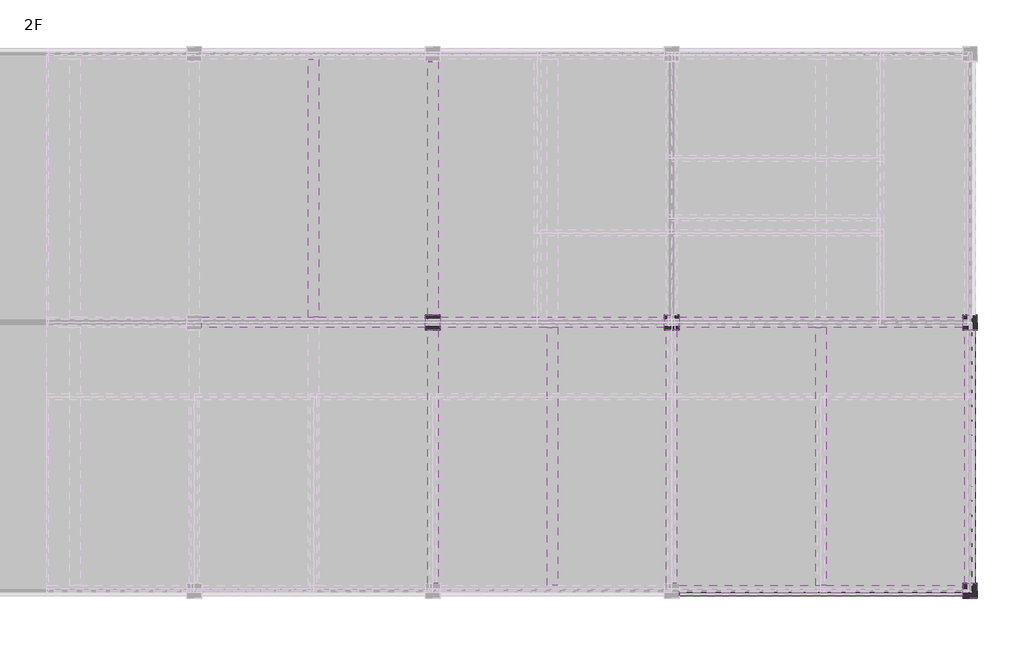
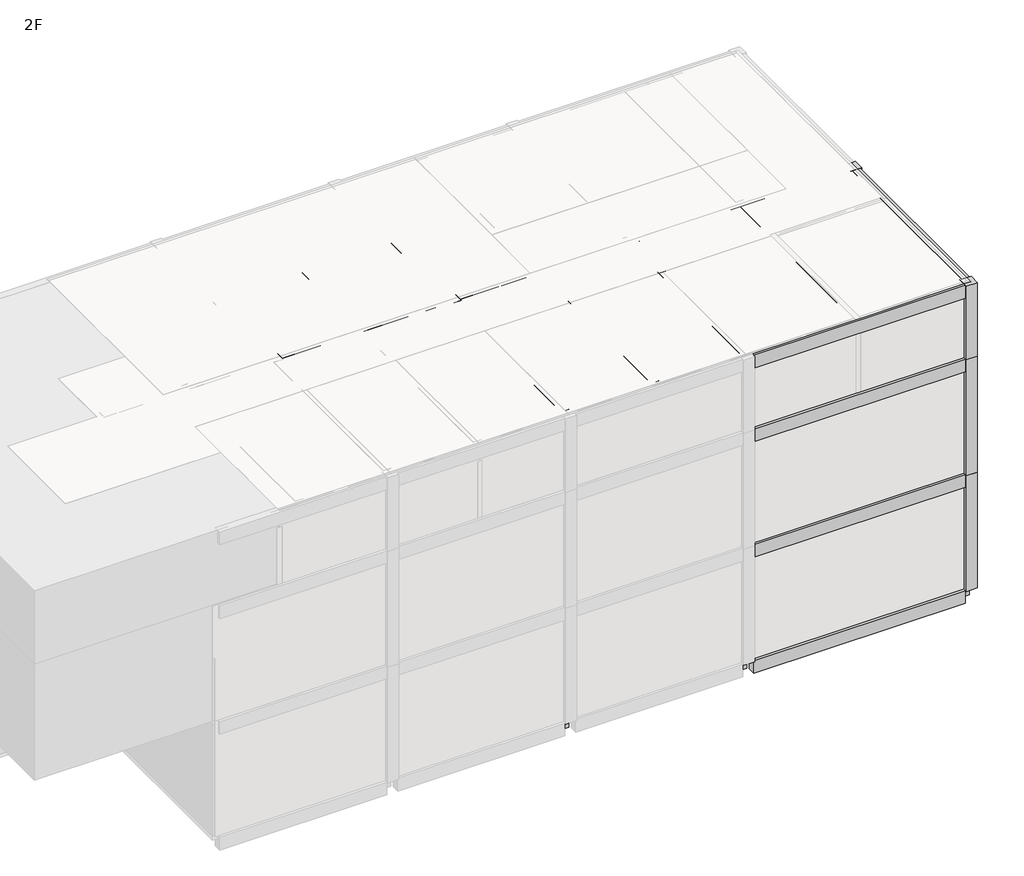
# One storey, part 6 of 7: 44 beams, 12 columns.
"""IFC4 building model written with IfcOpenShell, lengths in millimetres."""

from ifc_helpers import new_model, si_unit, frame, origin, place, context, project, spatial, polyline, outline, extrude, faceted_brep, element, save

model = new_model("IFC4")

# Units and contexts
model_context = context("Model", 3, world=origin())
ifc_project = project(units=[si_unit("LENGTHUNIT", "METRE", prefix="MILLI")], contexts=[model_context])

# Site, building, storey
site = spatial("IfcSite", under=ifc_project)
building = spatial("IfcBuilding", under=site)
storey = spatial("IfcBuildingStorey", under=building, Name="2F", Elevation=3500.0)

# Beams
placement = place(None, origin())
element("IfcBeam", 1, ObjectType="Concrete-Rectangular-Beam : BM111_400x500_RG1", at=placement, inside=storey, context=model_context, shape_type="SweptSolid", body=[
    extrude(outline(polyline([(65634.6521483, 173098.8614395), (65284.6521483, 173098.8614395), (65284.6521483, 181748.8614395), (65634.6521483, 181748.8614395), (65634.6521483, 173098.8614395)])), frame((0.0, 0.0, 2900.0), z_axis=(0.0, 0.0, 1.0), x_axis=(1.0, 0.0, 0.0)), (0.0, 0.0, 1.0), 600.0),
])
element("IfcBeam", 2, ObjectType="Concrete-Rectangular-Beam : BM111_400x500_RG1", at=placement, inside=storey, context=model_context, shape_type="SweptSolid", body=[
    extrude(outline(polyline([(73284.6521483, 172748.8614395), (73634.6521483, 172748.8614395), (73634.6521483, 164098.8614395), (73284.6521483, 164098.8614395), (73284.6521483, 172748.8614395)])), frame((0.0, 0.0, 2900.0), z_axis=(0.0, 0.0, 1.0), x_axis=(1.0, 0.0, 0.0)), (0.0, 0.0, 1.0), 600.0),
])
element("IfcBeam", 3, ObjectType="Concrete-Rectangular-Beam : BM111_400x500_RG1", at=placement, inside=storey, context=model_context, shape_type="SweptSolid", body=[
    extrude(outline(polyline([(82284.6521483, 172748.8614395), (82634.6521483, 172748.8614395), (82634.6521483, 164098.8614395), (82284.6521483, 164098.8614395), (82284.6521483, 172748.8614395)])), frame((0.0, 0.0, 2900.0), z_axis=(0.0, 0.0, 1.0), x_axis=(1.0, 0.0, 0.0)), (0.0, 0.0, 1.0), 600.0),
])
element("IfcBeam", 4, ObjectType="Concrete-Rectangular-Beam : BM111_400x500_RG1", at=placement, inside=storey, context=model_context, shape_type="SweptSolid", body=[
    extrude(outline(polyline([(65634.6521483, 173098.8614395), (65284.6521483, 173098.8614395), (65284.6521483, 181748.8614395), (65634.6521483, 181748.8614395), (65634.6521483, 173098.8614395)])), frame((0.0, 0.0, 8400.0), z_axis=(0.0, 0.0, 1.0), x_axis=(1.0, 0.0, 0.0)), (0.0, 0.0, 1.0), 600.0),
])
element("IfcBeam", 5, ObjectType="Concrete-Rectangular-Beam : BM111_400x500_RG1", at=placement, inside=storey, context=model_context, shape_type="SweptSolid", body=[
    extrude(outline(polyline([(73284.6521483, 172748.8614395), (73634.6521483, 172748.8614395), (73634.6521483, 164098.8614395), (73284.6521483, 164098.8614395), (73284.6521483, 172748.8614395)])), frame((0.0, 0.0, 8400.0), z_axis=(0.0, 0.0, 1.0), x_axis=(1.0, 0.0, 0.0)), (0.0, 0.0, 1.0), 600.0),
])
element("IfcBeam", 6, ObjectType="Concrete-Rectangular-Beam : BM111_400x500_RG1", at=placement, inside=storey, context=model_context, shape_type="SweptSolid", body=[
    extrude(outline(polyline([(82284.6521483, 172748.8614395), (82634.6521483, 172748.8614395), (82634.6521483, 164098.8614395), (82284.6521483, 164098.8614395), (82284.6521483, 172748.8614395)])), frame((0.0, 0.0, 8400.0), z_axis=(0.0, 0.0, 1.0), x_axis=(1.0, 0.0, 0.0)), (0.0, 0.0, 1.0), 600.0),
])
element("IfcBeam", 7, ObjectType="Concrete-Rectangular-Beam : BM111_400x500_RG1", at=placement, inside=storey, context=model_context, shape_type="SweptSolid", body=[
    extrude(outline(polyline([(65634.6521483, 173098.8614395), (65284.6521483, 173098.8614395), (65284.6521483, 181748.8614395), (65634.6521483, 181748.8614395), (65634.6521483, 173098.8614395)])), frame((0.0, 0.0, 13900.0), z_axis=(0.0, 0.0, 1.0), x_axis=(1.0, 0.0, 0.0)), (0.0, 0.0, 1.0), 600.0),
])
element("IfcBeam", 8, ObjectType="Concrete-Rectangular-Beam : BM111_400x500_RG1", at=placement, inside=storey, context=model_context, shape_type="SweptSolid", body=[
    extrude(outline(polyline([(73284.6521483, 172748.8614395), (73634.6521483, 172748.8614395), (73634.6521483, 164098.8614395), (73284.6521483, 164098.8614395), (73284.6521483, 172748.8614395)])), frame((0.0, 0.0, 13900.0), z_axis=(0.0, 0.0, 1.0), x_axis=(1.0, 0.0, 0.0)), (0.0, 0.0, 1.0), 600.0),
])
element("IfcBeam", 9, ObjectType="Concrete-Rectangular-Beam : BM111_400x500_RG1", at=placement, inside=storey, context=model_context, shape_type="SweptSolid", body=[
    extrude(outline(polyline([(82284.6521483, 172748.8614395), (82634.6521483, 172748.8614395), (82634.6521483, 164098.8614395), (82284.6521483, 164098.8614395), (82284.6521483, 172748.8614395)])), frame((0.0, 0.0, 13900.0), z_axis=(0.0, 0.0, 1.0), x_axis=(1.0, 0.0, 0.0)), (0.0, 0.0, 1.0), 600.0),
])
element("IfcBeam", 10, ObjectType="Concrete-Rectangular-Beam : BM111_400x500_RG1", at=placement, inside=storey, context=model_context, shape_type="SweptSolid", body=[
    extrude(outline(polyline([(65634.6521483, 173098.8614395), (65284.6521483, 173098.8614395), (65284.6521483, 181748.8614395), (65634.6521483, 181748.8614395), (65634.6521483, 173098.8614395)])), frame((0.0, 0.0, 17400.0), z_axis=(0.0, 0.0, 1.0), x_axis=(1.0, 0.0, 0.0)), (0.0, 0.0, 1.0), 600.0),
])
element("IfcBeam", 11, ObjectType="Concrete-Rectangular-Beam : BM111_400x500_RG1", at=placement, inside=storey, context=model_context, shape_type="SweptSolid", body=[
    extrude(outline(polyline([(73284.6521483, 172748.8614395), (73634.6521483, 172748.8614395), (73634.6521483, 164098.8614395), (73284.6521483, 164098.8614395), (73284.6521483, 172748.8614395)])), frame((0.0, 0.0, 17400.0), z_axis=(0.0, 0.0, 1.0), x_axis=(1.0, 0.0, 0.0)), (0.0, 0.0, 1.0), 600.0),
])
element("IfcBeam", 12, ObjectType="Concrete-Rectangular-Beam : BM111_400x500_RG1", at=placement, inside=storey, context=model_context, shape_type="SweptSolid", body=[
    extrude(outline(polyline([(82284.6521483, 172748.8614395), (82634.6521483, 172748.8614395), (82634.6521483, 164098.8614395), (82284.6521483, 164098.8614395), (82284.6521483, 172748.8614395)])), frame((0.0, 0.0, 17400.0), z_axis=(0.0, 0.0, 1.0), x_axis=(1.0, 0.0, 0.0)), (0.0, 0.0, 1.0), 600.0),
])
element("IfcBeam", 13, ObjectType="Concrete-Rectangular-Beam : BM111_400x500_RG1", at=placement, inside=storey, context=model_context, shape_type="Brep", body=[
    faceted_brep([(61709.6521483, 173098.8614395, 3500.0), (61709.6521483, 172748.8614395, 3500.0), (65284.6521483, 172748.8614395, 3500.0), (65634.6521483, 172748.8614395, 3500.0), (69209.6521483, 172748.8614395, 3500.0), (69209.6521483, 173098.8614395, 3500.0), (65634.6521483, 173098.8614395, 3500.0), (65284.6521483, 173098.8614395, 3500.0), (61709.6521483, 172748.8614395, 2900.0), (65284.6521483, 172748.8614395, 2900.0), (65634.6521483, 172748.8614395, 2900.0), (69209.6521483, 172748.8614395, 2900.0), (61709.6521483, 173098.8614395, 2900.0), (65284.6521483, 173098.8614395, 2900.0), (65634.6521483, 173098.8614395, 2900.0), (69209.6521483, 173098.8614395, 2900.0)], [[[0, 1, 2, 3, 4, 5, 6, 7]], [[1, 8, 9, 10, 11, 4, 3, 2]], [[8, 12, 13, 14, 15, 11, 10, 9]], [[12, 0, 7, 6, 5, 15, 14, 13]], [[1, 0, 12, 8]], [[5, 4, 11, 15]]]),
])
element("IfcBeam", 14, ObjectType="Concrete-Rectangular-Beam : BM111_400x500_RG1", at=placement, inside=storey, context=model_context, shape_type="Brep", body=[
    faceted_brep([(69709.6521483, 173098.8614395, 3500.0), (69709.6521483, 172748.8614395, 3500.0), (73284.6521483, 172748.8614395, 3500.0), (73634.6521483, 172748.8614395, 3500.0), (77209.6521483, 172748.8614395, 3500.0), (77209.6521483, 173098.8614395, 3500.0), (73634.6521483, 173098.8614395, 3500.0), (73284.6521483, 173098.8614395, 3500.0), (69709.6521483, 172748.8614395, 2900.0), (73284.6521483, 172748.8614395, 2900.0), (73634.6521483, 172748.8614395, 2900.0), (77209.6521483, 172748.8614395, 2900.0), (69709.6521483, 173098.8614395, 2900.0), (73284.6521483, 173098.8614395, 2900.0), (73634.6521483, 173098.8614395, 2900.0), (77209.6521483, 173098.8614395, 2900.0)], [[[0, 1, 2, 3, 4, 5, 6, 7]], [[1, 8, 9, 10, 11, 4, 3, 2]], [[8, 12, 13, 14, 15, 11, 10, 9]], [[12, 0, 7, 6, 5, 15, 14, 13]], [[1, 0, 12, 8]], [[5, 4, 11, 15]]]),
])
element("IfcBeam", 15, ObjectType="Concrete-Rectangular-Beam : BM111_400x500_RG1", at=placement, inside=storey, context=model_context, shape_type="Brep", body=[
    faceted_brep([(77709.6521483, 173098.8614395, 3500.0), (77709.6521483, 172748.8614395, 3500.0), (82284.6521483, 172748.8614395, 3500.0), (82634.6521483, 172748.8614395, 3500.0), (87209.6521483, 172748.8614395, 3500.0), (87209.6521483, 173098.8614395, 3500.0), (82634.6521483, 173098.8614395, 3500.0), (82284.6521483, 173098.8614395, 3500.0), (77709.6521483, 172748.8614395, 2900.0), (82284.6521483, 172748.8614395, 2900.0), (82634.6521483, 172748.8614395, 2900.0), (87209.6521483, 172748.8614395, 2900.0), (77709.6521483, 173098.8614395, 2900.0), (82284.6521483, 173098.8614395, 2900.0), (82634.6521483, 173098.8614395, 2900.0), (87209.6521483, 173098.8614395, 2900.0)], [[[0, 1, 2, 3, 4, 5, 6, 7]], [[1, 8, 9, 10, 11, 4, 3, 2]], [[8, 12, 13, 14, 15, 11, 10, 9]], [[12, 0, 7, 6, 5, 15, 14, 13]], [[1, 0, 12, 8]], [[5, 4, 11, 15]]]),
])
element("IfcBeam", 16, ObjectType="Concrete-Rectangular-Beam : BM111_400x500_RG1", at=placement, inside=storey, context=model_context, shape_type="Brep", body=[
    faceted_brep([(77709.6521483, 164098.8614395, 3500.0), (77709.6521483, 163748.8614395, 3500.0), (87209.6521483, 163748.8614395, 3500.0), (87209.6521483, 164098.8614395, 3500.0), (82634.6521483, 164098.8614395, 3500.0), (82284.6521483, 164098.8614395, 3500.0), (77709.6521483, 163748.8614395, 2900.0), (87209.6521483, 163748.8614395, 2900.0), (77709.6521483, 164098.8614395, 2900.0), (82284.6521483, 164098.8614395, 2900.0), (82634.6521483, 164098.8614395, 2900.0), (87209.6521483, 164098.8614395, 2900.0)], [[[0, 1, 2, 3, 4, 5]], [[1, 6, 7, 2]], [[6, 8, 9, 10, 11, 7]], [[8, 0, 5, 4, 3, 11, 10, 9]], [[1, 0, 8, 6]], [[3, 2, 7, 11]]]),
])
element("IfcBeam", 17, ObjectType="Concrete-Rectangular-Beam : BM111_400x500_RG1", at=placement, inside=storey, context=model_context, shape_type="Brep", body=[
    faceted_brep([(61709.6521483, 173098.8614395, 9000.0), (61709.6521483, 172748.8614395, 9000.0), (65284.6521483, 172748.8614395, 9000.0), (65634.6521483, 172748.8614395, 9000.0), (69209.6521483, 172748.8614395, 9000.0), (69209.6521483, 173098.8614395, 9000.0), (65634.6521483, 173098.8614395, 9000.0), (65284.6521483, 173098.8614395, 9000.0), (61709.6521483, 172748.8614395, 8400.0), (65284.6521483, 172748.8614395, 8400.0), (65634.6521483, 172748.8614395, 8400.0), (69209.6521483, 172748.8614395, 8400.0), (61709.6521483, 173098.8614395, 8400.0), (65284.6521483, 173098.8614395, 8400.0), (65634.6521483, 173098.8614395, 8400.0), (69209.6521483, 173098.8614395, 8400.0)], [[[0, 1, 2, 3, 4, 5, 6, 7]], [[1, 8, 9, 10, 11, 4, 3, 2]], [[8, 12, 13, 14, 15, 11, 10, 9]], [[12, 0, 7, 6, 5, 15, 14, 13]], [[1, 0, 12, 8]], [[5, 4, 11, 15]]]),
])
element("IfcBeam", 18, ObjectType="Concrete-Rectangular-Beam : BM111_400x500_RG1", at=placement, inside=storey, context=model_context, shape_type="Brep", body=[
    faceted_brep([(69709.6521483, 173098.8614395, 9000.0), (69709.6521483, 172748.8614395, 9000.0), (73284.6521483, 172748.8614395, 9000.0), (73634.6521483, 172748.8614395, 9000.0), (77209.6521483, 172748.8614395, 9000.0), (77209.6521483, 173098.8614395, 9000.0), (73634.6521483, 173098.8614395, 9000.0), (73284.6521483, 173098.8614395, 9000.0), (69709.6521483, 172748.8614395, 8400.0), (73284.6521483, 172748.8614395, 8400.0), (73634.6521483, 172748.8614395, 8400.0), (77209.6521483, 172748.8614395, 8400.0), (69709.6521483, 173098.8614395, 8400.0), (73284.6521483, 173098.8614395, 8400.0), (73634.6521483, 173098.8614395, 8400.0), (77209.6521483, 173098.8614395, 8400.0)], [[[0, 1, 2, 3, 4, 5, 6, 7]], [[1, 8, 9, 10, 11, 4, 3, 2]], [[8, 12, 13, 14, 15, 11, 10, 9]], [[12, 0, 7, 6, 5, 15, 14, 13]], [[1, 0, 12, 8]], [[5, 4, 11, 15]]]),
])
element("IfcBeam", 19, ObjectType="Concrete-Rectangular-Beam : BM111_400x500_RG1", at=placement, inside=storey, context=model_context, shape_type="Brep", body=[
    faceted_brep([(77709.6521483, 173098.8614395, 9000.0), (77709.6521483, 172748.8614395, 9000.0), (82284.6521483, 172748.8614395, 9000.0), (82634.6521483, 172748.8614395, 9000.0), (87209.6521483, 172748.8614395, 9000.0), (87209.6521483, 173098.8614395, 9000.0), (82634.6521483, 173098.8614395, 9000.0), (82284.6521483, 173098.8614395, 9000.0), (77709.6521483, 172748.8614395, 8400.0), (82284.6521483, 172748.8614395, 8400.0), (82634.6521483, 172748.8614395, 8400.0), (87209.6521483, 172748.8614395, 8400.0), (77709.6521483, 173098.8614395, 8400.0), (82284.6521483, 173098.8614395, 8400.0), (82634.6521483, 173098.8614395, 8400.0), (87209.6521483, 173098.8614395, 8400.0)], [[[0, 1, 2, 3, 4, 5, 6, 7]], [[1, 8, 9, 10, 11, 4, 3, 2]], [[8, 12, 13, 14, 15, 11, 10, 9]], [[12, 0, 7, 6, 5, 15, 14, 13]], [[1, 0, 12, 8]], [[5, 4, 11, 15]]]),
])
element("IfcBeam", 20, ObjectType="Concrete-Rectangular-Beam : BM111_400x500_RG1", at=placement, inside=storey, context=model_context, shape_type="Brep", body=[
    faceted_brep([(77709.6521483, 164098.8614395, 9000.0), (77709.6521483, 163748.8614395, 9000.0), (87209.6521483, 163748.8614395, 9000.0), (87209.6521483, 164098.8614395, 9000.0), (82634.6521483, 164098.8614395, 9000.0), (82284.6521483, 164098.8614395, 9000.0), (77709.6521483, 163748.8614395, 8400.0), (87209.6521483, 163748.8614395, 8400.0), (77709.6521483, 164098.8614395, 8400.0), (82284.6521483, 164098.8614395, 8400.0), (82634.6521483, 164098.8614395, 8400.0), (87209.6521483, 164098.8614395, 8400.0)], [[[0, 1, 2, 3, 4, 5]], [[1, 6, 7, 2]], [[6, 8, 9, 10, 11, 7]], [[8, 0, 5, 4, 3, 11, 10, 9]], [[1, 0, 8, 6]], [[3, 2, 7, 11]]]),
])
element("IfcBeam", 21, ObjectType="Concrete-Rectangular-Beam : BM111_400x500_RG1", at=placement, inside=storey, context=model_context, shape_type="Brep", body=[
    faceted_brep([(61709.6521483, 173098.8614395, 14500.0), (61709.6521483, 172748.8614395, 14500.0), (65284.6521483, 172748.8614395, 14500.0), (65634.6521483, 172748.8614395, 14500.0), (69209.6521483, 172748.8614395, 14500.0), (69209.6521483, 173098.8614395, 14500.0), (65634.6521483, 173098.8614395, 14500.0), (65284.6521483, 173098.8614395, 14500.0), (61709.6521483, 172748.8614395, 13900.0), (65284.6521483, 172748.8614395, 13900.0), (65634.6521483, 172748.8614395, 13900.0), (69209.6521483, 172748.8614395, 13900.0), (61709.6521483, 173098.8614395, 13900.0), (65284.6521483, 173098.8614395, 13900.0), (65634.6521483, 173098.8614395, 13900.0), (69209.6521483, 173098.8614395, 13900.0)], [[[0, 1, 2, 3, 4, 5, 6, 7]], [[1, 8, 9, 10, 11, 4, 3, 2]], [[8, 12, 13, 14, 15, 11, 10, 9]], [[12, 0, 7, 6, 5, 15, 14, 13]], [[1, 0, 12, 8]], [[5, 4, 11, 15]]]),
])
element("IfcBeam", 22, ObjectType="Concrete-Rectangular-Beam : BM111_400x500_RG1", at=placement, inside=storey, context=model_context, shape_type="Brep", body=[
    faceted_brep([(69709.6521483, 173098.8614395, 14500.0), (69709.6521483, 172748.8614395, 14500.0), (73284.6521483, 172748.8614395, 14500.0), (73634.6521483, 172748.8614395, 14500.0), (77209.6521483, 172748.8614395, 14500.0), (77209.6521483, 173098.8614395, 14500.0), (73634.6521483, 173098.8614395, 14500.0), (73284.6521483, 173098.8614395, 14500.0), (69709.6521483, 172748.8614395, 13900.0), (73284.6521483, 172748.8614395, 13900.0), (73634.6521483, 172748.8614395, 13900.0), (77209.6521483, 172748.8614395, 13900.0), (69709.6521483, 173098.8614395, 13900.0), (73284.6521483, 173098.8614395, 13900.0), (73634.6521483, 173098.8614395, 13900.0), (77209.6521483, 173098.8614395, 13900.0)], [[[0, 1, 2, 3, 4, 5, 6, 7]], [[1, 8, 9, 10, 11, 4, 3, 2]], [[8, 12, 13, 14, 15, 11, 10, 9]], [[12, 0, 7, 6, 5, 15, 14, 13]], [[1, 0, 12, 8]], [[5, 4, 11, 15]]]),
])
element("IfcBeam", 23, ObjectType="Concrete-Rectangular-Beam : BM111_400x500_RG1", at=placement, inside=storey, context=model_context, shape_type="Brep", body=[
    faceted_brep([(77709.6521483, 173098.8614395, 14500.0), (77709.6521483, 172748.8614395, 14500.0), (82284.6521483, 172748.8614395, 14500.0), (82634.6521483, 172748.8614395, 14500.0), (87209.6521483, 172748.8614395, 14500.0), (87209.6521483, 173098.8614395, 14500.0), (82634.6521483, 173098.8614395, 14500.0), (82284.6521483, 173098.8614395, 14500.0), (77709.6521483, 172748.8614395, 13900.0), (82284.6521483, 172748.8614395, 13900.0), (82634.6521483, 172748.8614395, 13900.0), (87209.6521483, 172748.8614395, 13900.0), (77709.6521483, 173098.8614395, 13900.0), (82284.6521483, 173098.8614395, 13900.0), (82634.6521483, 173098.8614395, 13900.0), (87209.6521483, 173098.8614395, 13900.0)], [[[0, 1, 2, 3, 4, 5, 6, 7]], [[1, 8, 9, 10, 11, 4, 3, 2]], [[8, 12, 13, 14, 15, 11, 10, 9]], [[12, 0, 7, 6, 5, 15, 14, 13]], [[1, 0, 12, 8]], [[5, 4, 11, 15]]]),
])
element("IfcBeam", 24, ObjectType="Concrete-Rectangular-Beam : BM111_400x500_RG1", at=placement, inside=storey, context=model_context, shape_type="Brep", body=[
    faceted_brep([(77709.6521483, 164098.8614395, 14500.0), (77709.6521483, 163748.8614395, 14500.0), (87209.6521483, 163748.8614395, 14500.0), (87209.6521483, 164098.8614395, 14500.0), (82634.6521483, 164098.8614395, 14500.0), (82284.6521483, 164098.8614395, 14500.0), (77709.6521483, 163748.8614395, 13900.0), (87209.6521483, 163748.8614395, 13900.0), (77709.6521483, 164098.8614395, 13900.0), (82284.6521483, 164098.8614395, 13900.0), (82634.6521483, 164098.8614395, 13900.0), (87209.6521483, 164098.8614395, 13900.0)], [[[0, 1, 2, 3, 4, 5]], [[1, 6, 7, 2]], [[6, 8, 9, 10, 11, 7]], [[8, 0, 5, 4, 3, 11, 10, 9]], [[1, 0, 8, 6]], [[3, 2, 7, 11]]]),
])
element("IfcBeam", 25, ObjectType="Concrete-Rectangular-Beam : BM111_400x500_RG1", at=placement, inside=storey, context=model_context, shape_type="Brep", body=[
    faceted_brep([(61709.6521483, 173098.8614395, 18000.0), (61709.6521483, 172748.8614395, 18000.0), (65284.6521483, 172748.8614395, 18000.0), (65634.6521483, 172748.8614395, 18000.0), (69209.6521483, 172748.8614395, 18000.0), (69209.6521483, 173098.8614395, 18000.0), (65634.6521483, 173098.8614395, 18000.0), (65284.6521483, 173098.8614395, 18000.0), (61709.6521483, 172748.8614395, 17400.0), (65284.6521483, 172748.8614395, 17400.0), (65634.6521483, 172748.8614395, 17400.0), (69209.6521483, 172748.8614395, 17400.0), (61709.6521483, 173098.8614395, 17400.0), (65284.6521483, 173098.8614395, 17400.0), (65634.6521483, 173098.8614395, 17400.0), (69209.6521483, 173098.8614395, 17400.0)], [[[0, 1, 2, 3, 4, 5, 6, 7]], [[1, 8, 9, 10, 11, 4, 3, 2]], [[8, 12, 13, 14, 15, 11, 10, 9]], [[12, 0, 7, 6, 5, 15, 14, 13]], [[1, 0, 12, 8]], [[5, 4, 11, 15]]]),
])
element("IfcBeam", 26, ObjectType="Concrete-Rectangular-Beam : BM111_400x500_RG1", at=placement, inside=storey, context=model_context, shape_type="Brep", body=[
    faceted_brep([(69709.6521483, 173098.8614395, 18000.0), (69709.6521483, 172748.8614395, 18000.0), (73284.6521483, 172748.8614395, 18000.0), (73634.6521483, 172748.8614395, 18000.0), (77209.6521483, 172748.8614395, 18000.0), (77209.6521483, 173098.8614395, 18000.0), (73634.6521483, 173098.8614395, 18000.0), (73284.6521483, 173098.8614395, 18000.0), (69709.6521483, 172748.8614395, 17400.0), (73284.6521483, 172748.8614395, 17400.0), (73634.6521483, 172748.8614395, 17400.0), (77209.6521483, 172748.8614395, 17400.0), (69709.6521483, 173098.8614395, 17400.0), (73284.6521483, 173098.8614395, 17400.0), (73634.6521483, 173098.8614395, 17400.0), (77209.6521483, 173098.8614395, 17400.0)], [[[0, 1, 2, 3, 4, 5, 6, 7]], [[1, 8, 9, 10, 11, 4, 3, 2]], [[8, 12, 13, 14, 15, 11, 10, 9]], [[12, 0, 7, 6, 5, 15, 14, 13]], [[1, 0, 12, 8]], [[5, 4, 11, 15]]]),
])
element("IfcBeam", 27, ObjectType="Concrete-Rectangular-Beam : BM111_400x500_RG1", at=placement, inside=storey, context=model_context, shape_type="Brep", body=[
    faceted_brep([(77709.6521483, 173098.8614395, 18000.0), (77709.6521483, 172748.8614395, 18000.0), (82284.6521483, 172748.8614395, 18000.0), (82634.6521483, 172748.8614395, 18000.0), (87209.6521483, 172748.8614395, 18000.0), (87209.6521483, 173098.8614395, 18000.0), (82634.6521483, 173098.8614395, 18000.0), (82284.6521483, 173098.8614395, 18000.0), (77709.6521483, 172748.8614395, 17400.0), (82284.6521483, 172748.8614395, 17400.0), (82634.6521483, 172748.8614395, 17400.0), (87209.6521483, 172748.8614395, 17400.0), (77709.6521483, 173098.8614395, 17400.0), (82284.6521483, 173098.8614395, 17400.0), (82634.6521483, 173098.8614395, 17400.0), (87209.6521483, 173098.8614395, 17400.0)], [[[0, 1, 2, 3, 4, 5, 6, 7]], [[1, 8, 9, 10, 11, 4, 3, 2]], [[8, 12, 13, 14, 15, 11, 10, 9]], [[12, 0, 7, 6, 5, 15, 14, 13]], [[1, 0, 12, 8]], [[5, 4, 11, 15]]]),
])
element("IfcBeam", 28, ObjectType="Concrete-Rectangular-Beam : BM111_400x500_RG1", at=placement, inside=storey, context=model_context, shape_type="Brep", body=[
    faceted_brep([(77709.6521483, 164098.8614395, 18000.0), (77709.6521483, 163748.8614395, 18000.0), (87209.6521483, 163748.8614395, 18000.0), (87209.6521483, 164098.8614395, 18000.0), (82634.6521483, 164098.8614395, 18000.0), (82284.6521483, 164098.8614395, 18000.0), (77709.6521483, 163748.8614395, 17400.0), (87209.6521483, 163748.8614395, 17400.0), (77709.6521483, 164098.8614395, 17400.0), (82284.6521483, 164098.8614395, 17400.0), (82634.6521483, 164098.8614395, 17400.0), (87209.6521483, 164098.8614395, 17400.0)], [[[0, 1, 2, 3, 4, 5]], [[1, 6, 7, 2]], [[6, 8, 9, 10, 11, 7]], [[8, 0, 5, 4, 3, 11, 10, 9]], [[1, 0, 8, 6]], [[3, 2, 7, 11]]]),
])
element("IfcBeam", 29, ObjectType="Concrete-Rectangular-Beam : BM111_400x500_RG1", at=placement, inside=storey, context=model_context, shape_type="SweptSolid", body=[
    extrude(outline(polyline([(69284.6521483, 181673.8614395), (69634.6521483, 181673.8614395), (69634.6521483, 173173.8614395), (69284.6521483, 173173.8614395), (69284.6521483, 181673.8614395)])), frame((0.0, 0.0, 2900.0), z_axis=(0.0, 0.0, 1.0), x_axis=(1.0, 0.0, 0.0)), (0.0, 0.0, 1.0), 600.0),
])
element("IfcBeam", 30, ObjectType="Concrete-Rectangular-Beam : BM111_400x500_RG1", at=placement, inside=storey, context=model_context, shape_type="SweptSolid", body=[
    extrude(outline(polyline([(69284.6521483, 172673.8614395), (69634.6521483, 172673.8614395), (69634.6521483, 164173.8614395), (69284.6521483, 164173.8614395), (69284.6521483, 172673.8614395)])), frame((0.0, 0.0, 2900.0), z_axis=(0.0, 0.0, 1.0), x_axis=(1.0, 0.0, 0.0)), (0.0, 0.0, 1.0), 600.0),
])
element("IfcBeam", 31, ObjectType="Concrete-Rectangular-Beam : BM111_400x500_RG1", at=placement, inside=storey, context=model_context, shape_type="SweptSolid", body=[
    extrude(outline(polyline([(77284.6521483, 172673.8614395), (77634.6521483, 172673.8614395), (77634.6521483, 164173.8614395), (77284.6521483, 164173.8614395), (77284.6521483, 172673.8614395)])), frame((0.0, 0.0, 2900.0), z_axis=(0.0, 0.0, 1.0), x_axis=(1.0, 0.0, 0.0)), (0.0, 0.0, 1.0), 600.0),
])
element("IfcBeam", 32, ObjectType="Concrete-Rectangular-Beam : BM111_400x500_RG1", at=placement, inside=storey, context=model_context, shape_type="SweptSolid", body=[
    extrude(outline(polyline([(87284.6521483, 172673.8614395), (87634.6521483, 172673.8614395), (87634.6521483, 164173.8614395), (87284.6521483, 164173.8614395), (87284.6521483, 172673.8614395)])), frame((0.0, 0.0, 2900.0), z_axis=(0.0, 0.0, 1.0), x_axis=(1.0, 0.0, 0.0)), (0.0, 0.0, 1.0), 600.0),
])
element("IfcBeam", 33, ObjectType="Concrete-Rectangular-Beam : BM111_400x500_RG1", at=placement, inside=storey, context=model_context, shape_type="SweptSolid", body=[
    extrude(outline(polyline([(69284.6521483, 181673.8614395), (69634.6521483, 181673.8614395), (69634.6521483, 173173.8614395), (69284.6521483, 173173.8614395), (69284.6521483, 181673.8614395)])), frame((0.0, 0.0, 8400.0), z_axis=(0.0, 0.0, 1.0), x_axis=(1.0, 0.0, 0.0)), (0.0, 0.0, 1.0), 600.0),
])
element("IfcBeam", 34, ObjectType="Concrete-Rectangular-Beam : BM111_400x500_RG1", at=placement, inside=storey, context=model_context, shape_type="SweptSolid", body=[
    extrude(outline(polyline([(69284.6521483, 172673.8614395), (69634.6521483, 172673.8614395), (69634.6521483, 164173.8614395), (69284.6521483, 164173.8614395), (69284.6521483, 172673.8614395)])), frame((0.0, 0.0, 8400.0), z_axis=(0.0, 0.0, 1.0), x_axis=(1.0, 0.0, 0.0)), (0.0, 0.0, 1.0), 600.0),
])
element("IfcBeam", 35, ObjectType="Concrete-Rectangular-Beam : BM111_400x500_RG1", at=placement, inside=storey, context=model_context, shape_type="SweptSolid", body=[
    extrude(outline(polyline([(77284.6521483, 172673.8614395), (77634.6521483, 172673.8614395), (77634.6521483, 164173.8614395), (77284.6521483, 164173.8614395), (77284.6521483, 172673.8614395)])), frame((0.0, 0.0, 8400.0), z_axis=(0.0, 0.0, 1.0), x_axis=(1.0, 0.0, 0.0)), (0.0, 0.0, 1.0), 600.0),
])
element("IfcBeam", 36, ObjectType="Concrete-Rectangular-Beam : BM111_400x500_RG1", at=placement, inside=storey, context=model_context, shape_type="SweptSolid", body=[
    extrude(outline(polyline([(87284.6521483, 172673.8614395), (87634.6521483, 172673.8614395), (87634.6521483, 164173.8614395), (87284.6521483, 164173.8614395), (87284.6521483, 172673.8614395)])), frame((0.0, 0.0, 8400.0), z_axis=(0.0, 0.0, 1.0), x_axis=(1.0, 0.0, 0.0)), (0.0, 0.0, 1.0), 600.0),
])
element("IfcBeam", 37, ObjectType="Concrete-Rectangular-Beam : BM111_400x500_RG1", at=placement, inside=storey, context=model_context, shape_type="SweptSolid", body=[
    extrude(outline(polyline([(69284.6521483, 181673.8614395), (69634.6521483, 181673.8614395), (69634.6521483, 173173.8614395), (69284.6521483, 173173.8614395), (69284.6521483, 181673.8614395)])), frame((0.0, 0.0, 13900.0), z_axis=(0.0, 0.0, 1.0), x_axis=(1.0, 0.0, 0.0)), (0.0, 0.0, 1.0), 600.0),
])
element("IfcBeam", 38, ObjectType="Concrete-Rectangular-Beam : BM111_400x500_RG1", at=placement, inside=storey, context=model_context, shape_type="SweptSolid", body=[
    extrude(outline(polyline([(69284.6521483, 172673.8614395), (69634.6521483, 172673.8614395), (69634.6521483, 164173.8614395), (69284.6521483, 164173.8614395), (69284.6521483, 172673.8614395)])), frame((0.0, 0.0, 13900.0), z_axis=(0.0, 0.0, 1.0), x_axis=(1.0, 0.0, 0.0)), (0.0, 0.0, 1.0), 600.0),
])
element("IfcBeam", 39, ObjectType="Concrete-Rectangular-Beam : BM111_400x500_RG1", at=placement, inside=storey, context=model_context, shape_type="SweptSolid", body=[
    extrude(outline(polyline([(77284.6521483, 172673.8614395), (77634.6521483, 172673.8614395), (77634.6521483, 164173.8614395), (77284.6521483, 164173.8614395), (77284.6521483, 172673.8614395)])), frame((0.0, 0.0, 13900.0), z_axis=(0.0, 0.0, 1.0), x_axis=(1.0, 0.0, 0.0)), (0.0, 0.0, 1.0), 600.0),
])
element("IfcBeam", 40, ObjectType="Concrete-Rectangular-Beam : BM111_400x500_RG1", at=placement, inside=storey, context=model_context, shape_type="SweptSolid", body=[
    extrude(outline(polyline([(87284.6521483, 172673.8614395), (87634.6521483, 172673.8614395), (87634.6521483, 164173.8614395), (87284.6521483, 164173.8614395), (87284.6521483, 172673.8614395)])), frame((0.0, 0.0, 13900.0), z_axis=(0.0, 0.0, 1.0), x_axis=(1.0, 0.0, 0.0)), (0.0, 0.0, 1.0), 600.0),
])
element("IfcBeam", 41, ObjectType="Concrete-Rectangular-Beam : BM111_400x500_RG1", at=placement, inside=storey, context=model_context, shape_type="SweptSolid", body=[
    extrude(outline(polyline([(69284.6521483, 181673.8614395), (69634.6521483, 181673.8614395), (69634.6521483, 173173.8614395), (69284.6521483, 173173.8614395), (69284.6521483, 181673.8614395)])), frame((0.0, 0.0, 17400.0), z_axis=(0.0, 0.0, 1.0), x_axis=(1.0, 0.0, 0.0)), (0.0, 0.0, 1.0), 600.0),
])
element("IfcBeam", 42, ObjectType="Concrete-Rectangular-Beam : BM111_400x500_RG1", at=placement, inside=storey, context=model_context, shape_type="SweptSolid", body=[
    extrude(outline(polyline([(69284.6521483, 172673.8614395), (69634.6521483, 172673.8614395), (69634.6521483, 164173.8614395), (69284.6521483, 164173.8614395), (69284.6521483, 172673.8614395)])), frame((0.0, 0.0, 17400.0), z_axis=(0.0, 0.0, 1.0), x_axis=(1.0, 0.0, 0.0)), (0.0, 0.0, 1.0), 600.0),
])
element("IfcBeam", 43, ObjectType="Concrete-Rectangular-Beam : BM111_400x500_RG1", at=placement, inside=storey, context=model_context, shape_type="SweptSolid", body=[
    extrude(outline(polyline([(77284.6521483, 172673.8614395), (77634.6521483, 172673.8614395), (77634.6521483, 164173.8614395), (77284.6521483, 164173.8614395), (77284.6521483, 172673.8614395)])), frame((0.0, 0.0, 17400.0), z_axis=(0.0, 0.0, 1.0), x_axis=(1.0, 0.0, 0.0)), (0.0, 0.0, 1.0), 600.0),
])
element("IfcBeam", 44, ObjectType="Concrete-Rectangular-Beam : BM111_400x500_RG1", at=placement, inside=storey, context=model_context, shape_type="SweptSolid", body=[
    extrude(outline(polyline([(87284.6521483, 172673.8614395), (87634.6521483, 172673.8614395), (87634.6521483, 164173.8614395), (87284.6521483, 164173.8614395), (87284.6521483, 172673.8614395)])), frame((0.0, 0.0, 17400.0), z_axis=(0.0, 0.0, 1.0), x_axis=(1.0, 0.0, 0.0)), (0.0, 0.0, 1.0), 600.0),
])

# Columns
element("IfcColumn", 45, ObjectType="Concrete-Rectangular-Column : CL111_500x500", at=placement, inside=storey, context=model_context, shape_type="Brep", body=[
    faceted_brep([(69709.6521483, 173173.8614395, 3500.0), (69709.6521483, 172673.8614395, 3500.0), (69209.6521483, 172673.8614395, 3500.0), (69209.6521483, 173173.8614395, 3500.0), (69709.6521483, 173173.8614395, 9000.0), (69709.6521483, 173098.8614395, 9000.0), (69709.6521483, 172748.8614395, 9000.0), (69709.6521483, 172673.8614395, 9000.0), (69634.6521483, 172673.8614395, 9000.0), (69284.6521483, 172673.8614395, 9000.0), (69209.6521483, 172673.8614395, 9000.0), (69209.6521483, 172748.8614395, 9000.0), (69209.6521483, 173098.8614395, 9000.0), (69209.6521483, 173173.8614395, 9000.0), (69284.6521483, 173173.8614395, 9000.0), (69634.6521483, 173173.8614395, 9000.0)], [[[0, 1, 2, 3]], [[4, 5, 6, 7, 1, 0]], [[7, 8, 9, 10, 2, 1]], [[10, 11, 12, 13, 3, 2]], [[13, 14, 15, 4, 0, 3]], [[4, 15, 14, 13, 12, 11, 10, 9, 8, 7, 6, 5]]]),
])
element("IfcColumn", 46, ObjectType="Concrete-Rectangular-Column : CL111_500x500", at=placement, inside=storey, context=model_context, shape_type="Brep", body=[
    faceted_brep([(69709.6521483, 173173.8614395, 9000.0), (69709.6521483, 172673.8614395, 9000.0), (69209.6521483, 172673.8614395, 9000.0), (69209.6521483, 173173.8614395, 9000.0), (69709.6521483, 173173.8614395, 14500.0), (69709.6521483, 173098.8614395, 14500.0), (69709.6521483, 172748.8614395, 14500.0), (69709.6521483, 172673.8614395, 14500.0), (69634.6521483, 172673.8614395, 14500.0), (69284.6521483, 172673.8614395, 14500.0), (69209.6521483, 172673.8614395, 14500.0), (69209.6521483, 172748.8614395, 14500.0), (69209.6521483, 173098.8614395, 14500.0), (69209.6521483, 173173.8614395, 14500.0), (69284.6521483, 173173.8614395, 14500.0), (69634.6521483, 173173.8614395, 14500.0)], [[[0, 1, 2, 3]], [[4, 5, 6, 7, 1, 0]], [[7, 8, 9, 10, 2, 1]], [[10, 11, 12, 13, 3, 2]], [[13, 14, 15, 4, 0, 3]], [[4, 15, 14, 13, 12, 11, 10, 9, 8, 7, 6, 5]]]),
])
element("IfcColumn", 47, ObjectType="Concrete-Rectangular-Column : CL111_500x500", at=placement, inside=storey, context=model_context, shape_type="Brep", body=[
    faceted_brep([(69709.6521483, 173173.8614395, 14500.0), (69709.6521483, 172673.8614395, 14500.0), (69209.6521483, 172673.8614395, 14500.0), (69209.6521483, 173173.8614395, 14500.0), (69709.6521483, 173173.8614395, 18000.0), (69709.6521483, 173098.8614395, 18000.0), (69709.6521483, 172748.8614395, 18000.0), (69709.6521483, 172673.8614395, 18000.0), (69634.6521483, 172673.8614395, 18000.0), (69284.6521483, 172673.8614395, 18000.0), (69209.6521483, 172673.8614395, 18000.0), (69209.6521483, 172748.8614395, 18000.0), (69209.6521483, 173098.8614395, 18000.0), (69209.6521483, 173173.8614395, 18000.0), (69284.6521483, 173173.8614395, 18000.0), (69634.6521483, 173173.8614395, 18000.0)], [[[0, 1, 2, 3]], [[4, 5, 6, 7, 1, 0]], [[7, 8, 9, 10, 2, 1]], [[10, 11, 12, 13, 3, 2]], [[13, 14, 15, 4, 0, 3]], [[4, 15, 14, 13, 12, 11, 10, 9, 8, 7, 6, 5]]]),
])
element("IfcColumn", 48, ObjectType="Concrete-Rectangular-Column : CL111_500x500", at=placement, inside=storey, context=model_context, shape_type="Brep", body=[
    faceted_brep([(77709.6521483, 173173.8614395, 3500.0), (77709.6521483, 172673.8614395, 3500.0), (77209.6521483, 172673.8614395, 3500.0), (77209.6521483, 173173.8614395, 3500.0), (77709.6521483, 173173.8614395, 9000.0), (77709.6521483, 173098.8614395, 9000.0), (77709.6521483, 172748.8614395, 9000.0), (77709.6521483, 172673.8614395, 9000.0), (77634.6521483, 172673.8614395, 9000.0), (77284.6521483, 172673.8614395, 9000.0), (77209.6521483, 172673.8614395, 9000.0), (77209.6521483, 172748.8614395, 9000.0), (77209.6521483, 173098.8614395, 9000.0), (77209.6521483, 173173.8614395, 9000.0), (77284.6521483, 173173.8614395, 9000.0), (77634.6521483, 173173.8614395, 9000.0)], [[[0, 1, 2, 3]], [[4, 5, 6, 7, 1, 0]], [[7, 8, 9, 10, 2, 1]], [[10, 11, 12, 13, 3, 2]], [[13, 14, 15, 4, 0, 3]], [[4, 15, 14, 13, 12, 11, 10, 9, 8, 7, 6, 5]]]),
])
element("IfcColumn", 49, ObjectType="Concrete-Rectangular-Column : CL111_500x500", at=placement, inside=storey, context=model_context, shape_type="Brep", body=[
    faceted_brep([(77709.6521483, 173173.8614395, 9000.0), (77709.6521483, 172673.8614395, 9000.0), (77209.6521483, 172673.8614395, 9000.0), (77209.6521483, 173173.8614395, 9000.0), (77709.6521483, 173173.8614395, 14500.0), (77709.6521483, 173098.8614395, 14500.0), (77709.6521483, 172748.8614395, 14500.0), (77709.6521483, 172673.8614395, 14500.0), (77634.6521483, 172673.8614395, 14500.0), (77284.6521483, 172673.8614395, 14500.0), (77209.6521483, 172673.8614395, 14500.0), (77209.6521483, 172748.8614395, 14500.0), (77209.6521483, 173098.8614395, 14500.0), (77209.6521483, 173173.8614395, 14500.0), (77284.6521483, 173173.8614395, 14500.0), (77634.6521483, 173173.8614395, 14500.0)], [[[0, 1, 2, 3]], [[4, 5, 6, 7, 1, 0]], [[7, 8, 9, 10, 2, 1]], [[10, 11, 12, 13, 3, 2]], [[13, 14, 15, 4, 0, 3]], [[4, 15, 14, 13, 12, 11, 10, 9, 8, 7, 6, 5]]]),
])
element("IfcColumn", 50, ObjectType="Concrete-Rectangular-Column : CL111_500x500", at=placement, inside=storey, context=model_context, shape_type="Brep", body=[
    faceted_brep([(77709.6521483, 173173.8614395, 14500.0), (77709.6521483, 172673.8614395, 14500.0), (77209.6521483, 172673.8614395, 14500.0), (77209.6521483, 173173.8614395, 14500.0), (77709.6521483, 173173.8614395, 18000.0), (77709.6521483, 173098.8614395, 18000.0), (77709.6521483, 172748.8614395, 18000.0), (77709.6521483, 172673.8614395, 18000.0), (77634.6521483, 172673.8614395, 18000.0), (77284.6521483, 172673.8614395, 18000.0), (77209.6521483, 172673.8614395, 18000.0), (77209.6521483, 172748.8614395, 18000.0), (77209.6521483, 173098.8614395, 18000.0), (77209.6521483, 173173.8614395, 18000.0), (77284.6521483, 173173.8614395, 18000.0), (77634.6521483, 173173.8614395, 18000.0)], [[[0, 1, 2, 3]], [[4, 5, 6, 7, 1, 0]], [[7, 8, 9, 10, 2, 1]], [[10, 11, 12, 13, 3, 2]], [[13, 14, 15, 4, 0, 3]], [[4, 15, 14, 13, 12, 11, 10, 9, 8, 7, 6, 5]]]),
])
element("IfcColumn", 51, ObjectType="Concrete-Rectangular-Column : CL111_500x500", at=placement, inside=storey, context=model_context, shape_type="Brep", body=[
    faceted_brep([(87709.6521483, 173173.8614395, 3500.0), (87709.6521483, 172673.8614395, 3500.0), (87209.6521483, 172673.8614395, 3500.0), (87209.6521483, 173173.8614395, 3500.0), (87709.6521483, 173173.8614395, 9000.0), (87709.6521483, 172673.8614395, 9000.0), (87634.6521483, 172673.8614395, 9000.0), (87284.6521483, 172673.8614395, 9000.0), (87209.6521483, 172673.8614395, 9000.0), (87209.6521483, 172748.8614395, 9000.0), (87209.6521483, 173098.8614395, 9000.0), (87209.6521483, 173173.8614395, 9000.0), (87284.6521483, 173173.8614395, 9000.0), (87634.6521483, 173173.8614395, 9000.0)], [[[0, 1, 2, 3]], [[4, 5, 1, 0]], [[5, 6, 7, 8, 2, 1]], [[8, 9, 10, 11, 3, 2]], [[11, 12, 13, 4, 0, 3]], [[4, 13, 12, 11, 10, 9, 8, 7, 6, 5]]]),
])
element("IfcColumn", 52, ObjectType="Concrete-Rectangular-Column : CL111_500x500", at=placement, inside=storey, context=model_context, shape_type="Brep", body=[
    faceted_brep([(87709.6521483, 173173.8614395, 9000.0), (87709.6521483, 172673.8614395, 9000.0), (87209.6521483, 172673.8614395, 9000.0), (87209.6521483, 173173.8614395, 9000.0), (87709.6521483, 173173.8614395, 14500.0), (87709.6521483, 172673.8614395, 14500.0), (87634.6521483, 172673.8614395, 14500.0), (87284.6521483, 172673.8614395, 14500.0), (87209.6521483, 172673.8614395, 14500.0), (87209.6521483, 172748.8614395, 14500.0), (87209.6521483, 173098.8614395, 14500.0), (87209.6521483, 173173.8614395, 14500.0), (87284.6521483, 173173.8614395, 14500.0), (87634.6521483, 173173.8614395, 14500.0)], [[[0, 1, 2, 3]], [[4, 5, 1, 0]], [[5, 6, 7, 8, 2, 1]], [[8, 9, 10, 11, 3, 2]], [[11, 12, 13, 4, 0, 3]], [[4, 13, 12, 11, 10, 9, 8, 7, 6, 5]]]),
])
element("IfcColumn", 53, ObjectType="Concrete-Rectangular-Column : CL111_500x500", at=placement, inside=storey, context=model_context, shape_type="Brep", body=[
    faceted_brep([(87709.6521483, 173173.8614395, 14500.0), (87709.6521483, 172673.8614395, 14500.0), (87209.6521483, 172673.8614395, 14500.0), (87209.6521483, 173173.8614395, 14500.0), (87709.6521483, 173173.8614395, 18000.0), (87709.6521483, 172673.8614395, 18000.0), (87634.6521483, 172673.8614395, 18000.0), (87284.6521483, 172673.8614395, 18000.0), (87209.6521483, 172673.8614395, 18000.0), (87209.6521483, 172748.8614395, 18000.0), (87209.6521483, 173098.8614395, 18000.0), (87209.6521483, 173173.8614395, 18000.0), (87284.6521483, 173173.8614395, 18000.0), (87634.6521483, 173173.8614395, 18000.0)], [[[0, 1, 2, 3]], [[4, 5, 1, 0]], [[5, 6, 7, 8, 2, 1]], [[8, 9, 10, 11, 3, 2]], [[11, 12, 13, 4, 0, 3]], [[4, 13, 12, 11, 10, 9, 8, 7, 6, 5]]]),
])
element("IfcColumn", 54, ObjectType="Concrete-Rectangular-Column : CL111_500x500", at=placement, inside=storey, context=model_context, shape_type="Brep", body=[
    faceted_brep([(87709.6521483, 164173.8614395, 3500.0), (87709.6521483, 163673.8614395, 3500.0), (87209.6521483, 163673.8614395, 3500.0), (87209.6521483, 164173.8614395, 3500.0), (87709.6521483, 164173.8614395, 9000.0), (87709.6521483, 163673.8614395, 9000.0), (87209.6521483, 163673.8614395, 9000.0), (87209.6521483, 163748.8614395, 9000.0), (87209.6521483, 164098.8614395, 9000.0), (87209.6521483, 164173.8614395, 9000.0), (87284.6521483, 164173.8614395, 9000.0), (87634.6521483, 164173.8614395, 9000.0)], [[[0, 1, 2, 3]], [[4, 5, 1, 0]], [[5, 6, 2, 1]], [[6, 7, 8, 9, 3, 2]], [[9, 10, 11, 4, 0, 3]], [[4, 11, 10, 9, 8, 7, 6, 5]]]),
])
element("IfcColumn", 55, ObjectType="Concrete-Rectangular-Column : CL111_500x500", at=placement, inside=storey, context=model_context, shape_type="Brep", body=[
    faceted_brep([(87709.6521483, 164173.8614395, 9000.0), (87709.6521483, 163673.8614395, 9000.0), (87209.6521483, 163673.8614395, 9000.0), (87209.6521483, 164173.8614395, 9000.0), (87709.6521483, 164173.8614395, 14500.0), (87709.6521483, 163673.8614395, 14500.0), (87209.6521483, 163673.8614395, 14500.0), (87209.6521483, 163748.8614395, 14500.0), (87209.6521483, 164098.8614395, 14500.0), (87209.6521483, 164173.8614395, 14500.0), (87284.6521483, 164173.8614395, 14500.0), (87634.6521483, 164173.8614395, 14500.0)], [[[0, 1, 2, 3]], [[4, 5, 1, 0]], [[5, 6, 2, 1]], [[6, 7, 8, 9, 3, 2]], [[9, 10, 11, 4, 0, 3]], [[4, 11, 10, 9, 8, 7, 6, 5]]]),
])
element("IfcColumn", 56, ObjectType="Concrete-Rectangular-Column : CL111_500x500", at=placement, inside=storey, context=model_context, shape_type="Brep", body=[
    faceted_brep([(87709.6521483, 164173.8614395, 14500.0), (87709.6521483, 163673.8614395, 14500.0), (87209.6521483, 163673.8614395, 14500.0), (87209.6521483, 164173.8614395, 14500.0), (87709.6521483, 164173.8614395, 18000.0), (87709.6521483, 163673.8614395, 18000.0), (87209.6521483, 163673.8614395, 18000.0), (87209.6521483, 163748.8614395, 18000.0), (87209.6521483, 164098.8614395, 18000.0), (87209.6521483, 164173.8614395, 18000.0), (87284.6521483, 164173.8614395, 18000.0), (87634.6521483, 164173.8614395, 18000.0)], [[[0, 1, 2, 3]], [[4, 5, 1, 0]], [[5, 6, 2, 1]], [[6, 7, 8, 9, 3, 2]], [[9, 10, 11, 4, 0, 3]], [[4, 11, 10, 9, 8, 7, 6, 5]]]),
])

save(model, "model.ifc")

# Revit data of these elements
# Type "Concrete-Rectangular-Beam : BM111_400x500_RG1"
#   중앙부 하부근 = "3-D20"
#   중앙부 상부근 = "3-D20"
#   중앙부 보조근 = ""
#   중앙부 늑근 = "2-D10 @200"
#   외단부 하부근 = "3-D20"
#   외단부 상부근 = "3-D20"
#   외단부 보조근 = ""
#   외단부 늑근 = "2-D10 @100"
#   부호 = "RG1"
#   내단부 하부근 = "3-D20"
#   내단부 상부근 = "3-D20"
#   내단부 보조근 = ""
#   내단부 늑근 = "2-D10 @100"
#   ALL 하부근 = ""
#   ALL 상부근 = ""
#   ALL 보조근 = ""
#   ALL 늑근 = ""
#   Width = 400 mm
#   Height = 500 mm
#   Length [instance default] = 1524 mm
#   Structural Material [instance default] = 콘크리트 - 현장타설 콘크리트
#   hec_material3 [instance default] = none
#   hec_material2 [instance default] = none
#   hec_material1 [instance default] = none
#   Assembly Code = ""
# Type "Concrete-Rectangular-Column : CL111_500x500"
#   Description = "UG 철골 기둥용 Pedestal"
#   b = 500 mm
#   h = 500 mm
#   hec_material3 [instance default] = none
#   hec_material2 [instance default] = A03AE056-00001_Bitumen/Bituminous/Asphalt Coating
#   hec_material1 [instance default] = A03AC035-00001_Form Work (3 times in use)_Flat
#   Structural Material [instance default] = A03AC032-00007_Structural Concrete_Type1_25MPa-30Mpa
# Elements 1, 2, 3, 4, 5, 6, 7, 8, 9, 10, 11, 12, 13, 14, 15, 16, 17, 18, 19, 20, 21, 22, 23, 24, 25, 26, 27, 28, 29, 30, 31, 32, 33, 34, 35, 36, 37, 38, 39, 40, 41, 42, 43, 44 (IfcBeam, "Concrete-Rectangular-Beam : BM111_400x500_RG1")
#   Comments = ""
#   hec_material3 = none
#   hec_material2 = none
#   hec_material1 = none
#   Structural Material = 콘크리트 - 현장타설 콘크리트
#   Phase Created = New Construction
#   Materials on its faces: "콘크리트 - 현장타설 콘크리트"
# Elements 45, 46, 47, 48, 49, 50, 51, 52, 53, 54, 55, 56 (IfcColumn, "Concrete-Rectangular-Column : CL111_500x500")
#   Comments = ""
#   hec_material3 = none
#   hec_material2 = none
#   hec_material1 = none
#   Structural Material = 콘크리트 - 현장타설 콘크리트
#   Phase Created = New Construction
#   Materials on its faces: "콘크리트 - 현장타설 콘크리트"
# Materials
#   "콘크리트 - 현장타설 콘크리트": class "콘크리트", colour RGB 192 192 192, transparency 0
#   "A03AE056-00001_Bitumen/Bituminous/Asphalt Coating": class "Generic", colour RGB 17 17 17, transparency 0, Description = "Damp-proofing", W00) Work Master Code = "A03AE056-00001", W01) Work Master_Lv1 = "Concrete Work", W02) Work Master_Lv2 = "Concrete Protective Coating (U/G)", W03) Work Master_Spec.1 = "Bitumen/Bituminous/Asphalt Coating", Cost = 0
#   "A03AC035-00001_Form Work (3 times in use)_Flat": class "Wood", colour RGB 149 120 74, transparency 0, Description = "Plywood", W00) Work Master Code = "A03AC035-00001", W01) Work Master_Lv1 = "Concrete Work", W02) Work Master_Lv2 = "Substructure Work", W03) Work Master_Spec.1 = "Form Work (3 times in use)", W04) Work Master_Spec.2 = "Flat Form", W05) Work Master_Spec.3 = "Dressed Lumber, Plywood or Steel Form(Wood Planks are not Allowed) incl. Chamfer", Cost = 0
#   "A03AC032-00007_Structural Concrete_Type1_25MPa-30Mpa": class "Concrete", colour RGB 176 176 176, transparency 0, Keynote = "09910.A1", Description = "Reinf. Conc.", W00) Work Master Code = "A03AC032-00007", W01) Work Master_Lv1 = "Concrete Work", W02) Work Master_Lv2 = "Substructure Work", W03) Work Master_Spec.1 = "Structural Concrete", W04) Work Master_Spec.2 = "Cement Type-1", W05) Work Master_Spec.3 = "25MPa < F'c (Cylinder Strength) ≤ 30MPa", Cost = 0
